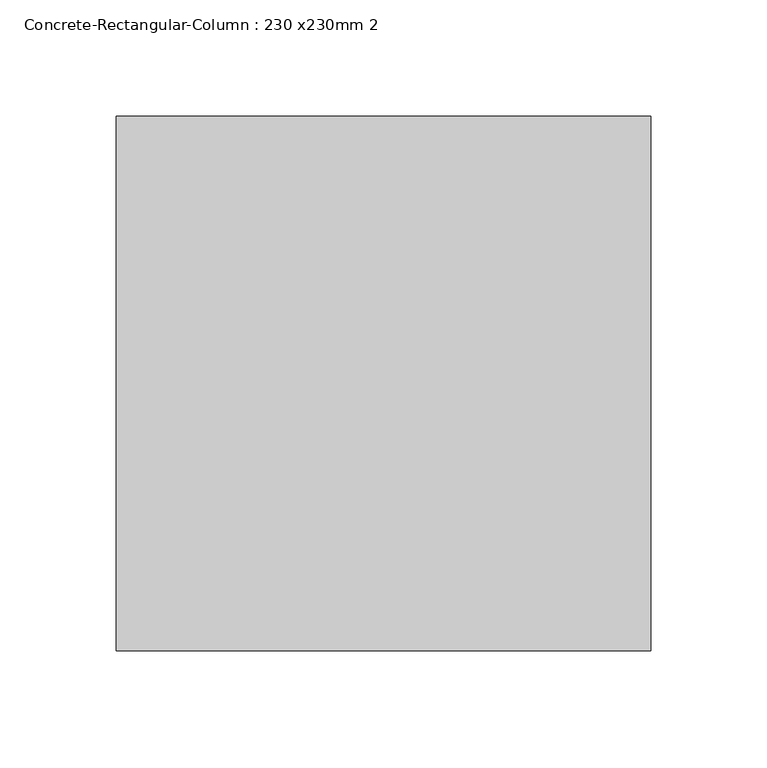
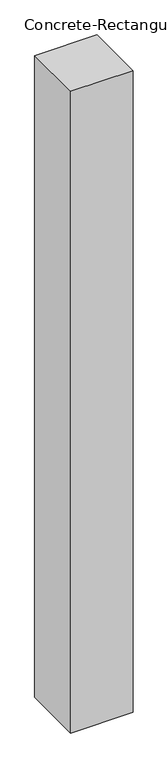
"""IFC4 building model written with IfcOpenShell, lengths in millimetres: column geometry, Concrete-Rectangular-Column : 230 x230mm 2."""

from ifc_helpers import new_model, si_unit, frame, origin, place, context, project, spatial, polyline, outline, extrude, source, transform, mapped, element, save


def concrete_rectangular_column_230_x230mm_2_460f90e7(model_context):
    return source(origin(), model_context, "Body", "SweptSolid", [
        extrude(outline(polyline([(115.0, 115.0), (115.0, -115.0), (-115.0, -115.0), (-115.0, 115.0), (115.0, 115.0)])), frame((0.0, 0.0, -2500.0), z_axis=(0.0, 0.0, 1.0), x_axis=(1.0, 0.0, 0.0)), (0.0, 0.0, 1.0), 2500.0),
    ])


if __name__ == "__main__":
    model = new_model("IFC4")
    model_context = context("Model", 3, world=origin())
    ifc_project = project(units=[si_unit("LENGTHUNIT", "METRE", prefix="MILLI")], contexts=[model_context])
    site = spatial("IfcSite", under=ifc_project)
    building = spatial("IfcBuilding", under=site)
    placement = place(None, origin())
    concrete_rectangular_column_230_x230mm_2_shape = concrete_rectangular_column_230_x230mm_2_460f90e7(model_context)
    element("IfcColumn", 1, ObjectType="Concrete-Rectangular-Column : 230 x230mm 2", at=placement, inside=building, context=model_context, shape_type="MappedRepresentation", body=[
        mapped(concrete_rectangular_column_230_x230mm_2_shape, transform((0.0, 0.0, 0.0), x_axis=(1.0, 0.0, 0.0), y_axis=(0.0, 1.0, 0.0), z_axis=(0.0, 0.0, 1.0))),
    ])
    save(model, "model.ifc")

# Revit data of these elements
# Type "Concrete-Rectangular-Column : 230 x230mm 2"
#   b = 230 mm
#   h = 230 mm
#   Structural Material [instance default] = Concrete, Cast-in-Place gray
# Element 1 (IfcColumn, "Concrete-Rectangular-Column : 230 x230mm 2")
#   Materials on its faces: "Concrete, Cast-in-Place gray"
# Materials
#   "Concrete, Cast-in-Place gray": class "Concrete", colour RGB 192 192 192, transparency 0, Description = "Cast-in-place concrete", Cost = 0
